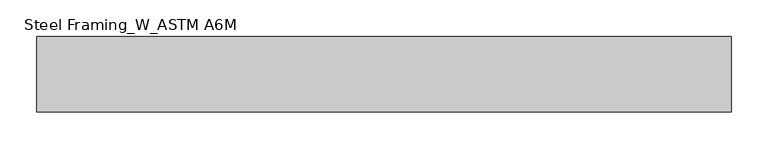
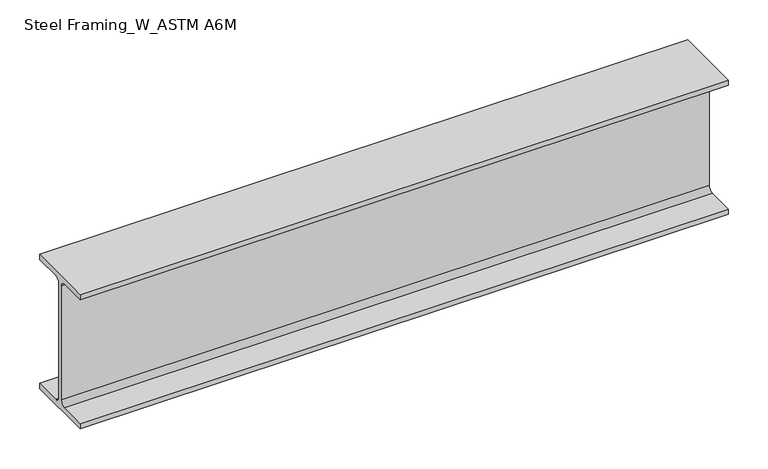
"""IFC4 building model written with IfcOpenShell, lengths in millimetres: beam geometry, Steel Framing_W_ASTM A6M : H_SB_AR_S02_W200x22.5_J1."""

from ifc_helpers import new_model, si_unit, point, frame, frame_2d, origin, place, context, project, spatial, polyline, circle_curve, trimmed, segment, composite_curve, outline, extrude, source, transform, mapped, element, save


def steel_framing_w_astm_a6m_f3cc38eb(model_context):
    return source(origin(), model_context, "Body", "SweptSolid", [
        extrude(outline(composite_curve([segment(polyline([(51.0, -95.0), (51.0, -103.0), (-51.0, -103.0), (-51.0, -95.0), (-10.71, -95.0)]), True, "CONTINUOUS"), segment(trimmed(circle_curve(frame_2d((-10.71, -87.4)), 7.6), [point((-10.71, -95.0))], [point((-3.11, -87.4))], True, "CARTESIAN"), True, "CONTINUOUS"), segment(polyline([(-3.11, -87.4), (-3.11, 87.4)]), True, "CONTINUOUS"), segment(trimmed(circle_curve(frame_2d((-10.71, 87.4)), 7.6), [point((-3.11, 87.4))], [point((-10.71, 95.0))], True, "CARTESIAN"), True, "CONTINUOUS"), segment(polyline([(-10.71, 95.0), (-51.0, 95.0), (-51.0, 103.0), (51.0, 103.0), (51.0, 95.0), (10.71, 95.0)]), True, "CONTINUOUS"), segment(trimmed(circle_curve(frame_2d((10.71, 87.4)), 7.6), [point((10.71, 95.0))], [point((3.11, 87.4))], True, "CARTESIAN"), True, "CONTINUOUS"), segment(polyline([(3.11, 87.4), (3.11, -87.4)]), True, "CONTINUOUS"), segment(trimmed(circle_curve(frame_2d((10.71, -87.4)), 7.6), [point((3.11, -87.4))], [point((10.71, -95.0))], True, "CARTESIAN"), True, "CONTINUOUS"), segment(polyline([(10.71, -95.0), (51.0, -95.0)]), True, "CONTINUOUS")], self_intersect=False)), frame((-470.3, 0.0, 0.0), z_axis=(1.0, 0.0, 0.0), x_axis=(0.0, 1.0, 0.0)), (0.0, 0.0, 1.0), 940.6),
    ])


if __name__ == "__main__":
    model = new_model("IFC4")
    model_context = context("Model", 3, world=origin())
    ifc_project = project(units=[si_unit("LENGTHUNIT", "METRE", prefix="MILLI")], contexts=[model_context])
    site = spatial("IfcSite", under=ifc_project)
    building = spatial("IfcBuilding", under=site)
    placement = place(None, origin())
    steel_framing_w_astm_a6m_shape = steel_framing_w_astm_a6m_f3cc38eb(model_context)
    element("IfcBeam", 1, ObjectType="Steel Framing_W_ASTM A6M : H_SB_AR_S02_W200x22.5_J1", at=placement, inside=building, context=model_context, shape_type="MappedRepresentation", body=[
        mapped(steel_framing_w_astm_a6m_shape, transform((0.0, 0.0, 0.0), x_axis=(1.0, 0.0, 0.0), y_axis=(0.0, 1.0, 0.0), z_axis=(0.0, 0.0, 1.0))),
    ])
    save(model, "model.ifc")

# Revit data of these elements
# Type "Steel Framing_W_ASTM A6M : H_SB_AR_S02_W200x22.5_J1"
#   Section Name Key = "W8x15"
#   Width = 10.2 cm
#   Web Thickness = 0.622 cm
#   Web Fillet = 0.76 cm
#   Warping Constant = 13900.0 cm⁶
#   Torsional Moment of Inertia = 5.70 cm⁴
#   Section Area = 28.6 cm²
#   Plastic Modulus weak axis = 43.8 cm³
#   Plastic Modulus strong axis = 223.0 cm³
#   Perimeter = 0.795 m²/m
#   Nominal Weight = 22.50 kgf/m
#   Moment of Inertia weak axis = 142.00 cm⁴
#   Moment of Inertia strong axis = 2000.00 cm⁴
#   Height = 20.6 cm
#   Flange Thickness = 0.8 cm
#   Elastic Modulus weak axis = 27.9 cm³
#   Elastic Modulus strong axis = 193.0 cm³
#   Centroid Vertical = 10.3 cm
#   Centroid Horizontal = 5.1 cm
#   Length [instance default] = 1500 mm
#   Structural Material [instance default] = Steel, 45-345
#   Bolt Spacing = 0
#   Assembly Code = ""
# Element 1 (IfcBeam, "Steel Framing_W_ASTM A6M : H_SB_AR_S02_W200x22.5_J1")
#   Materials on its faces: "Steel, 45-345"
# Materials
#   "Steel, 45-345": class "Metal", colour RGB 189 187 185, transparency 0, Description = "Steel 345 MPa", Cost = 0
